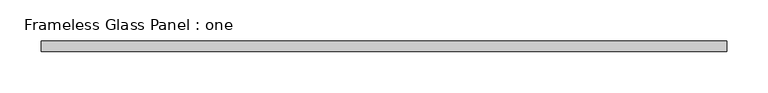
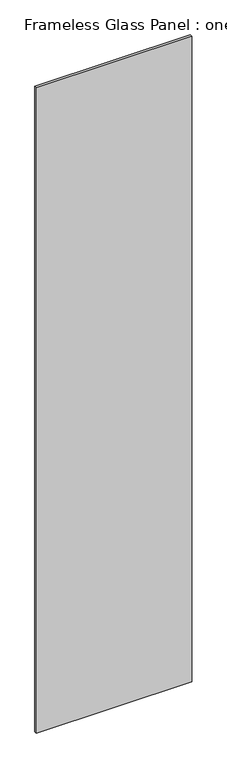
"""IFC4 building model written with IfcOpenShell, lengths in millimetres: plate geometry, Frameless Glass Panel : one."""

from ifc_helpers import new_model, si_unit, origin, origin_with_axes, place, context, project, spatial, polyline, outline, extrude, source, transform, mapped, element, save


def frameless_glass_panel_one_c2898315(model_context):
    return source(origin(), model_context, "Body", "SweptSolid", [
        extrude(outline(polyline([(416.3592749, -6.35), (-416.3592749, -6.35), (-416.3592749, 6.35), (416.3592749, 6.35), (416.3592749, -6.35)])), origin_with_axes(), (0.0, 0.0, 1.0), 3651.25),
    ])


if __name__ == "__main__":
    model = new_model("IFC4")
    model_context = context("Model", 3, world=origin())
    ifc_project = project(units=[si_unit("LENGTHUNIT", "METRE", prefix="MILLI")], contexts=[model_context])
    site = spatial("IfcSite", under=ifc_project)
    building = spatial("IfcBuilding", under=site)
    placement = place(None, origin())
    frameless_glass_panel_one_shape = frameless_glass_panel_one_c2898315(model_context)
    element("IfcPlate", 1, ObjectType="Frameless Glass Panel : one", at=placement, inside=building, context=model_context, shape_type="MappedRepresentation", body=[
        mapped(frameless_glass_panel_one_shape, transform((0.0, 0.0, 0.0), x_axis=(1.0, 0.0, 0.0), y_axis=(0.0, 1.0, 0.0), z_axis=(0.0, 0.0, 1.0))),
    ])
    save(model, "model.ifc")

# Revit data of these elements
# Type "Frameless Glass Panel : one"
#   Glass Thickness = 0' - 0 1/2"
#   Gap btwn Panels = 0' - 0 1/4"
#   Panel Material = TEMPERED GLASS DOOR/SIDELIGHT TO MATCH EXISTING CONF. ROOM
# Element 1 (IfcPlate, "Frameless Glass Panel : one")
#   Materials on its faces: "TEMPERED GLASS DOOR/SIDELIGHT TO MATCH EXISTING CONF. ROOM"
# Materials
#   "TEMPERED GLASS DOOR/SIDELIGHT TO MATCH EXISTING CONF. ROOM": class "Glass", colour RGB 218 227 224, transparency 0.85, Description = "Soda Lime Glass", Cost = 0
